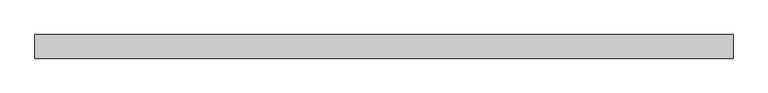
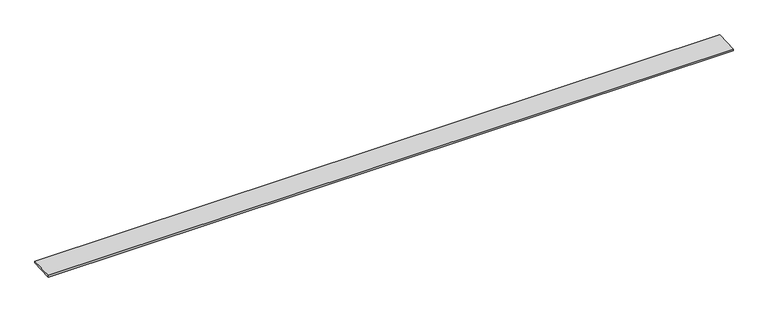
"""IFC4 building model written with IfcOpenShell, lengths in millimetres: proxy geometry, Generic Models 7:Generic Models 1:2:Generic Models 1:2 : Generic Models 7:Generic Models 1:337419:17 : Generic Models 7:Generic Models 1:2:Generic Models 1:2 : Generic Models 7:Generic Models 1:337419:306751."""

from ifc_helpers import new_model, si_unit, frame, origin, place, context, project, spatial, polyline, outline, extrude, source, transform, mapped, element, save


def generic_models_e4d2903c(model_context):
    return source(origin(), model_context, "Body", "SweptSolid", [
        extrude(outline(polyline([(0.0, -164.842211), (0.0, 0.0), (4876.8, 0.0), (4876.8, -164.842211), (0.0, -164.842211)])), frame((596182.8367239, -568180.8644202, 8562.4272903), z_axis=(0.0, -0.041630544767773385, 0.9991330730900356), x_axis=(-1.0, 0.0, 0.0)), (0.0, 0.0, 1.0), 12.7),
    ])


if __name__ == "__main__":
    model = new_model("IFC4")
    model_context = context("Model", 3, world=origin())
    ifc_project = project(units=[si_unit("LENGTHUNIT", "METRE", prefix="MILLI")], contexts=[model_context])
    site = spatial("IfcSite", under=ifc_project)
    building = spatial("IfcBuilding", under=site)
    placement = place(None, origin())
    generic_models_shape = generic_models_e4d2903c(model_context)
    element("IfcBuildingElementProxy", 1, Name="Generic Models 7:Generic Models 1:2:Generic Models 1:2 : Generic Models 7:Generic Models 1:337419:17 : Generic Models 7:Generic Models 1:2:Generic Models 1:2 : Generic Models 7:Generic Models 1:337419:306751", ObjectType="Generic Models 7:Generic Models 1:2:Generic Models 1:2 : Generic Models 7:Generic Models 1:337419:17 : Generic Models 7:Generic Models 1:2:Generic Models 1:2 : Generic Models 7:Generic Models 1:337419:306751", at=placement, inside=building, context=model_context, shape_type="MappedRepresentation", body=[
        mapped(generic_models_shape, transform((0.0, 0.0, 0.0), x_axis=(1.0, 0.0, 0.0), y_axis=(0.0, 1.0, 0.0), z_axis=(0.0, 0.0, 1.0))),
    ])
    save(model, "model.ifc")

# Revit data of these elements
# Type "Generic Models 7:Generic Models 1:2:Generic Models 1:2 : Generic Models 7:Generic Models 1:337419:17 : Generic Models 7:Generic Models 1:2:Generic Models 1:2 : Generic Models 7:Generic Models 1:337419:306751"
#   NameOverride = "Generic Models 7:Generic Models 1:2:Generic Models 1:2 : Generic Models 7:Generic Models 1:337419:306751"
#   ObjectTypeOverride = "Generic Models 1:2 : Generic Models 7:Generic Models 1:337419"
#   Reference = "Generic Models 1"
#   Tag = "306751"
# Element 1 (IfcBuildingElementProxy, "Generic Models 7:Generic Models 1:2:Generic Models 1:2 : Generic Models 7:Generic Models 1:337419:17 : Generic Models 7:Generic Models 1:2:Generic Models 1:2 : Generic Models 7:Generic Models 1:337419:306751")
#   Materials on its faces: "FIRE RETARDTANT WOOD BLOCKING - SIZE AS NEC."
# Materials
#   "FIRE RETARDTANT WOOD BLOCKING - SIZE AS NEC.": class "Wood", colour RGB 144 113 62, transparency 0, Description = "Pinus Echinata", Cost = 0
